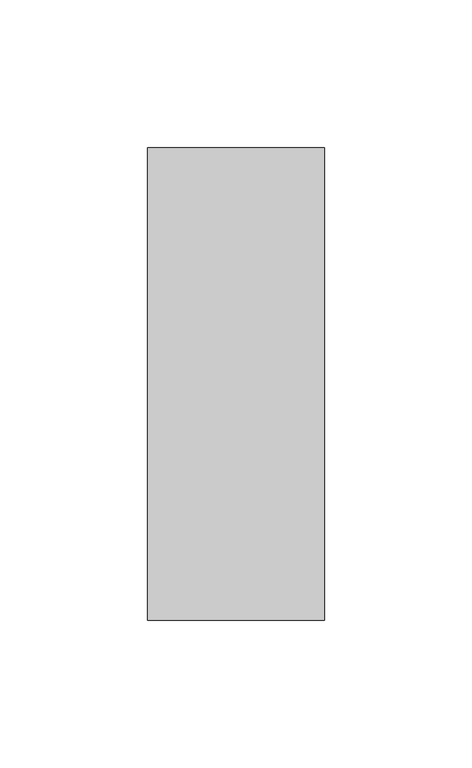
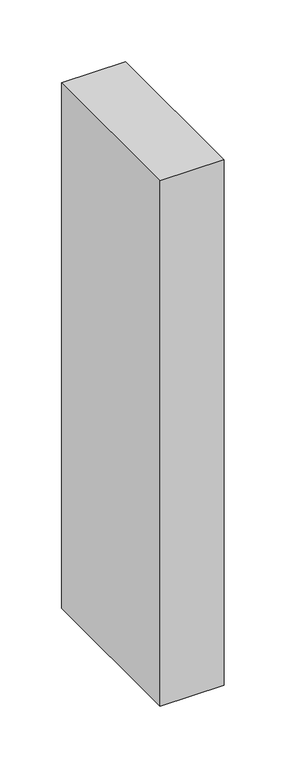
"""IFC4 building model written with IfcOpenShell, lengths in millimetres: column geometry, Madeira de lei-Coluna : Pontalete 6X16cm."""

from ifc_helpers import new_model, si_unit, frame, origin, place, context, project, spatial, polyline, outline, extrude, source, transform, mapped, element, save


def column_d0cf395a(model_context):
    return source(origin(), model_context, "Body", "SweptSolid", [
        extrude(outline(polyline([(30.0, 80.0), (30.0, -80.0), (-30.0, -80.0), (-30.0, 80.0), (30.0, 80.0)])), frame((0.0, 0.0, 6710.0), z_axis=(0.0, 0.0, 1.0), x_axis=(1.0, 0.0, 0.0)), (0.0, 0.0, 1.0), 520.0),
    ])


if __name__ == "__main__":
    model = new_model("IFC4")
    model_context = context("Model", 3, world=origin())
    ifc_project = project(units=[si_unit("LENGTHUNIT", "METRE", prefix="MILLI")], contexts=[model_context])
    site = spatial("IfcSite", under=ifc_project)
    building = spatial("IfcBuilding", under=site)
    placement = place(None, origin())
    column_shape = column_d0cf395a(model_context)
    element("IfcColumn", 1, ObjectType="Madeira de lei-Coluna : Pontalete 6X16cm", at=placement, inside=building, context=model_context, shape_type="MappedRepresentation", body=[
        mapped(column_shape, transform((0.0, 0.0, 0.0), x_axis=(1.0, 0.0, 0.0), y_axis=(0.0, 1.0, 0.0), z_axis=(0.0, 0.0, 1.0))),
    ])
    save(model, "model.ifc")

# Revit data of these elements
# Type "Madeira de lei-Coluna : Pontalete 6X16cm"
#   A = 0.01952 m²
#   b = 0.06 m
#   d = 0.16 m
#   Structural Material [instance default] = none
#   Assembly Code = ""
# Element 1 (IfcColumn, "Madeira de lei-Coluna : Pontalete 6X16cm")
#   Structural Material = .MADEIRAMENTO
#   Materials on its faces: ".MADEIRAMENTO"
# Materials
#   ".MADEIRAMENTO": class ".CC_MADEIRAS", colour RGB 212 179 113, transparency 0, Cost = 0
